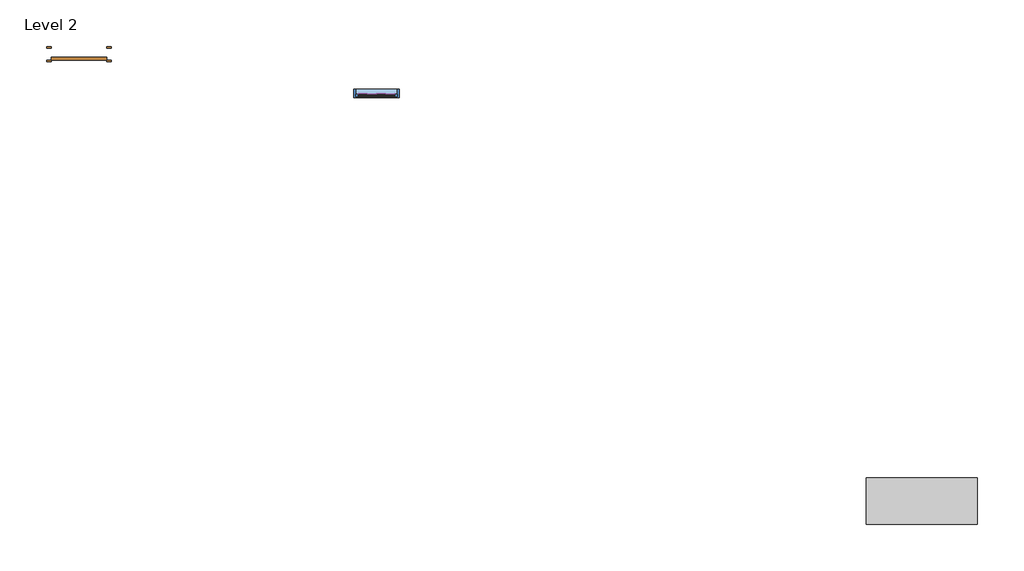
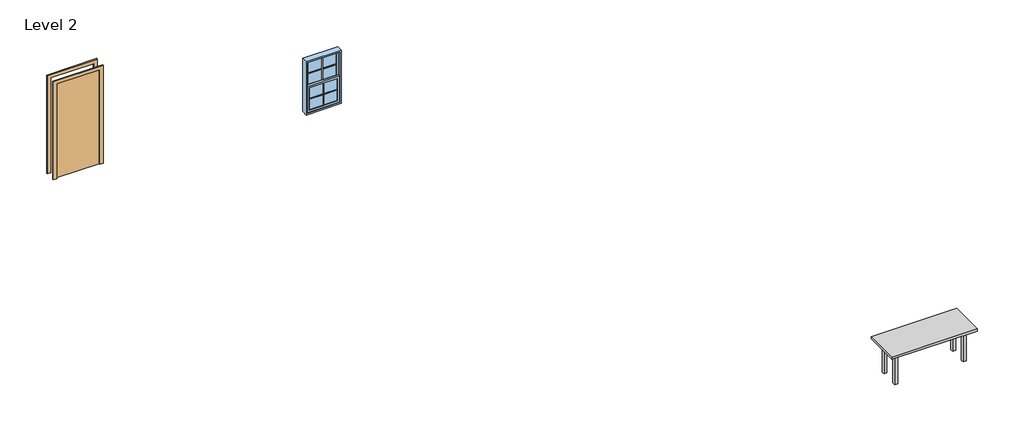
# One storey: 2 proxies, 1 door, 1 furniture element, 1 window.
"""IFC4 building model written with IfcOpenShell, lengths in millimetres."""

import ifcopenshell
import ifcopenshell.guid

model = None  # the IFC model being written
_history = None  # IfcOwnerHistory: only IFC2X3 demands one
_inside = {}  # id of a spatial element -> (the spatial element, [elements in it])
_under = {}  # id of a project, library or spatial element -> (it, [spatial elements below it])
_declared = {}  # id of a project -> (the project, [libraries it declares])
_typed = {}  # id of a type object -> (the type object, [elements of that type])
_made_of = {}  # id of a material, layer set ... -> (it, [elements and type objects made of it])


def new_model(schema):
    """Start an empty IFC model of exactly this schema.

    Asked for "IFC4X3", IfcOpenShell would pick the latest addendum, in which some entities
    have other attributes; the version numbers below select the first issue.
    IFC2X3 requires an IfcOwnerHistory on every rooted entity: one is made here for all.
    """
    global model, _history
    if schema == "IFC4X3":
        model = ifcopenshell.file(schema_version=(4, 3, 0, 0))
    else:
        model = ifcopenshell.file(schema=schema)
    _inside.clear()
    _under.clear()
    _declared.clear()
    _typed.clear()
    _made_of.clear()
    _history = None
    if model.schema == "IFC2X3":
        org = make("IfcOrganization", Name="unknown")
        user = make(
            "IfcPersonAndOrganization",
            ThePerson=make("IfcPerson", FamilyName="unknown"),
            TheOrganization=org,
        )
        app = make(
            "IfcApplication",
            ApplicationDeveloper=org,
            Version="unknown",
            ApplicationFullName="unknown",
            ApplicationIdentifier="unknown",
        )
        _history = make(
            "IfcOwnerHistory",
            OwningUser=user,
            OwningApplication=app,
            ChangeAction="ADDED",
            CreationDate=0,
        )
    return model


def make(cls, **values):
    """One entity of the class cls with the attributes given. An attribute that is None is left unset."""
    return model.create_entity(
        cls, **{name: value for name, value in values.items() if value is not None}
    )


def rooted(cls, **values):
    """An entity with a GlobalId (a new one), such as an element, a storey or a relation."""
    return make(cls, GlobalId=ifcopenshell.guid.new(), OwnerHistory=_history, **values)


def si_unit(unit_type, name, prefix=None):
    """IfcSIUnit, for example si_unit("LENGTHUNIT", "METRE", prefix="MILLI")."""
    return make("IfcSIUnit", UnitType=unit_type, Prefix=prefix, Name=name)


def assignment(units):
    """IfcUnitAssignment: the units of a project."""
    return None if units is None else make("IfcUnitAssignment", Units=units)


def point(xyz):
    """IfcCartesianPoint."""
    return None if xyz is None else make("IfcCartesianPoint", Coordinates=xyz)


def direction(xyz):
    """IfcDirection."""
    return None if xyz is None else make("IfcDirection", DirectionRatios=xyz)


def frame(location, z_axis=None, x_axis=None):
    """IfcAxis2Placement3D, a coordinate frame: its origin and axes. An axis left out is left unset."""
    return make(
        "IfcAxis2Placement3D",
        Location=point(location),
        Axis=direction(z_axis),
        RefDirection=direction(x_axis),
    )


def origin():
    """The frame at (0, 0, 0) with its axes left unset."""
    return frame((0.0, 0.0, 0.0))


def origin_with_axes():
    """The frame at (0, 0, 0) with the z axis (0, 0, 1) and the x axis (1, 0, 0) written out."""
    return frame((0.0, 0.0, 0.0), z_axis=(0.0, 0.0, 1.0), x_axis=(1.0, 0.0, 0.0))


def place(relative_to, where):
    """IfcLocalPlacement: puts the frame where relative to a parent placement (None: the world)."""
    return make(
        "IfcLocalPlacement", PlacementRelTo=relative_to, RelativePlacement=where
    )


def context(
    kind, dimensions, precision=None, world=None, true_north=None, identifier=None
):
    """IfcGeometricRepresentationContext, for example the 3D "Model" context."""
    return make(
        "IfcGeometricRepresentationContext",
        ContextIdentifier=identifier,
        ContextType=kind,
        CoordinateSpaceDimension=dimensions,
        Precision=precision,
        WorldCoordinateSystem=world,
        TrueNorth=true_north,
    )


def project(units=None, contexts=None):
    """IfcProject with its units and contexts."""
    return rooted(
        "IfcProject",
        Name="project",
        RepresentationContexts=contexts,
        UnitsInContext=assignment(units),
    )


def spatial(cls, under=None, at=None, **own):
    """A site, building, storey or space (cls), placed at a placement, below another one or the project."""
    s = rooted(cls, ObjectPlacement=at, **own)
    if under is not None:
        _under.setdefault(under.id(), (under, []))[1].append(s)
    return s


def polyline(points):
    """IfcPolyline through the points."""
    return make("IfcPolyline", Points=[point(p) for p in points])


def outline(outer, holes=None, kind="AREA"):
    """IfcArbitraryClosedProfileDef: a profile drawn as a closed curve; with holes, ...WithVoids."""
    if holes is None:
        return make("IfcArbitraryClosedProfileDef", ProfileType=kind, OuterCurve=outer)
    return make(
        "IfcArbitraryProfileDefWithVoids",
        ProfileType=kind,
        OuterCurve=outer,
        InnerCurves=holes,
    )


def extrude(swept, where, along, depth):
    """IfcExtrudedAreaSolid: the profile swept, set in the frame where, extruded along a direction by depth."""
    return make(
        "IfcExtrudedAreaSolid",
        SweptArea=swept,
        Position=where,
        ExtrudedDirection=direction(along),
        Depth=depth,
    )


def shape(context_of_items, identifier, shape_type, items):
    """IfcShapeRepresentation: the items that make up one representation, for example the "Body"."""
    return make(
        "IfcShapeRepresentation",
        ContextOfItems=context_of_items,
        RepresentationIdentifier=identifier,
        RepresentationType=shape_type,
        Items=items,
    )


def source(mapping_origin, context_of_items, identifier, shape_type, items):
    """IfcRepresentationMap: a shape defined once, which mapped items show again and again."""
    return make(
        "IfcRepresentationMap",
        MappingOrigin=mapping_origin,
        MappedRepresentation=shape(context_of_items, identifier, shape_type, items),
    )


def transform(
    local_origin,
    x_axis=None,
    y_axis=None,
    z_axis=None,
    scale=None,
    scale2=None,
    scale3=None,
    uniform=True,
):
    """IfcCartesianTransformationOperator3D, or its non-uniform kind. x_axis, y_axis, z_axis: its Axis1, 2, 3."""
    if uniform:
        return make(
            "IfcCartesianTransformationOperator3D",
            Axis1=direction(x_axis),
            Axis2=direction(y_axis),
            LocalOrigin=point(local_origin),
            Scale=scale,
            Axis3=direction(z_axis),
        )
    return make(
        "IfcCartesianTransformationOperator3DnonUniform",
        Axis1=direction(x_axis),
        Axis2=direction(y_axis),
        LocalOrigin=point(local_origin),
        Scale=scale,
        Axis3=direction(z_axis),
        Scale2=scale2,
        Scale3=scale3,
    )


def mapped(mapping_source, mapping_target):
    """IfcMappedItem: shows the shape of a source again, moved by a transform."""
    return make(
        "IfcMappedItem", MappingSource=mapping_source, MappingTarget=mapping_target
    )


def made_of(thing, what):
    """Note that an element or type object is made of a material, layer set ...; save() writes the relation."""
    if what is not None:
        _made_of.setdefault(what.id(), (what, []))[1].append(thing)
    return thing


def element(
    cls,
    number,
    at=None,
    inside=None,
    cuts=None,
    type_object=None,
    material=None,
    context=None,
    identifier="Body",
    shape_type=None,
    held_by="IfcProductDefinitionShape",
    body=None,
    shapes=None,
    **own,
):
    """One element of the class cls, such as IfcWall. Its Tag is "e" and its number.

    at: its placement. inside: the storey or other place that contains it. cuts: it is an
    opening in that element (IfcRelVoidsElement). A single representation is given by context,
    identifier, shape_type and body (its items); several are given by shapes. held_by: the class
    of the entity that holds the representations. save() writes the other relations.
    """
    e = rooted(cls, Tag="e%d" % number, ObjectPlacement=at, **own)
    if body is not None:
        shapes = [shape(context, identifier, shape_type, body)]
    if shapes is not None:
        e.Representation = make(held_by, Representations=shapes)
    if inside is not None:
        _inside.setdefault(inside.id(), (inside, []))[1].append(e)
    if cuts is not None:
        rooted(
            "IfcRelVoidsElement", RelatingBuildingElement=cuts, RelatedOpeningElement=e
        )
    if type_object is not None:
        _typed.setdefault(type_object.id(), (type_object, []))[1].append(e)
    return made_of(e, material)


def aggregate(whole, parts):
    """IfcRelAggregates: a whole, such as a stair, and the parts it consists of."""
    return rooted("IfcRelAggregates", RelatingObject=whole, RelatedObjects=parts)


def save(model, path):
    """Write the relations noted so far, then the file.

    IfcRelAggregates (storeys below a building ...), IfcRelContainedInSpatialStructure (elements
    in a storey), IfcRelDefinesByType, IfcRelAssociatesMaterial and IfcRelDeclares: one each for
    every whole, place, type object, material and project.
    """
    for whole, parts in _under.values():
        aggregate(whole, parts)
    for where, things in _inside.values():
        rooted(
            "IfcRelContainedInSpatialStructure",
            RelatedElements=things,
            RelatingStructure=where,
        )
    for kind, things in _typed.values():
        rooted("IfcRelDefinesByType", RelatedObjects=things, RelatingType=kind)
    for what, things in _made_of.values():
        rooted("IfcRelAssociatesMaterial", RelatedObjects=things, RelatingMaterial=what)
    for by, libraries in _declared.values():
        rooted("IfcRelDeclares", RelatingContext=by, RelatedDefinitions=libraries)
    model.write(path)


def m_muntin_pattern_2x2_m_muntin_pattern_2x2_aaec3afb(model_context):
    return source(origin(), model_context, "Body", "SweptSolid", [
        extrude(outline(polyline([(257.1375, -6.35), (257.1375, -298.8), (244.4375, -298.8), (244.4375, -6.35), (0.0, -6.35), (0.0, 6.35), (244.4375, 6.35), (244.4375, 298.8), (257.1375, 298.8), (257.1375, 6.35), (501.575, 6.35), (501.575, -6.35), (257.1375, -6.35)])), frame((0.0, 9.525, 0.0), z_axis=(0.0, 1.0, 0.0), x_axis=(0.0, 0.0, 1.0)), (0.0, 0.0, 1.0), 12.7),
        extrude(outline(polyline([(257.1375, -6.35), (257.1375, -298.8), (244.4375, -298.8), (244.4375, -6.35), (0.0, -6.35), (0.0, 6.35), (244.4375, 6.35), (244.4375, 298.8), (257.1375, 298.8), (257.1375, 6.35), (501.575, 6.35), (501.575, -6.35), (257.1375, -6.35)])), frame((0.0, -22.225, 0.0), z_axis=(0.0, 1.0, 0.0), x_axis=(0.0, 0.0, 1.0)), (0.0, 0.0, 1.0), 12.7),
    ])


def m_single_flush_0915_x_2134mm_6a9e8738(model_context):
    return source(origin(), model_context, "Body", "SweptSolid", [
        extrude(outline(polyline([(2210.0, -533.5), (0.0, -533.5), (0.0, -457.5), (2134.0, -457.5), (2134.0, 457.5), (0.0, 457.5), (0.0, 533.5), (2210.0, 533.5), (2210.0, -533.5)])), frame((0.0, 100.0, 0.0), z_axis=(0.0, 1.0, 0.0), x_axis=(0.0, 0.0, 1.0)), (0.0, 0.0, 1.0), 25.0),
        extrude(outline(polyline([(2210.0, 533.5), (2210.0, -533.5), (0.0, -533.5), (0.0, -457.5), (2134.0, -457.5), (2134.0, 457.5), (0.0, 457.5), (0.0, 533.5), (2210.0, 533.5)])), frame((0.0, -125.0, 0.0), z_axis=(0.0, 1.0, 0.0), x_axis=(0.0, 0.0, 1.0)), (0.0, 0.0, 1.0), 25.0),
        extrude(outline(polyline([(457.5, 49.0), (-457.5, 49.0), (-457.5, 100.0), (457.5, 100.0), (457.5, 49.0)])), origin_with_axes(), (0.0, 0.0, 1.0), 2134.0),
    ])


def m_table_rectangular_1830_x_0762mm_a0b3b7a0(model_context):
    return source(origin(), model_context, "Body", "SweptSolid", [
        extrude(outline(polyline([(699.1, 190.5), (699.1, 165.1), (-699.1, 165.1), (-699.1, 190.5), (699.1, 190.5)])), frame((0.0, 0.0, 609.6), z_axis=(0.0, 0.0, 1.0), x_axis=(1.0, 0.0, 0.0)), (0.0, 0.0, 1.0), 101.6),
        extrude(outline(polyline([(699.1, -190.5), (-699.1, -190.5), (-699.1, -165.1), (699.1, -165.1), (699.1, -190.5)])), frame((0.0, 0.0, 609.6), z_axis=(0.0, 0.0, 1.0), x_axis=(1.0, 0.0, 0.0)), (0.0, 0.0, 1.0), 101.6),
        extrude(outline(polyline([(-711.8, -165.1), (-737.2, -165.1), (-737.2, 165.1), (-711.8, 165.1), (-711.8, -165.1)])), frame((0.0, 0.0, 609.6), z_axis=(0.0, 0.0, 1.0), x_axis=(1.0, 0.0, 0.0)), (0.0, 0.0, 1.0), 101.6),
        extrude(outline(polyline([(711.8, -165.1), (711.8, 165.1), (737.2, 165.1), (737.2, -165.1), (711.8, -165.1)])), frame((0.0, 0.0, 609.6), z_axis=(0.0, 0.0, 1.0), x_axis=(1.0, 0.0, 0.0)), (0.0, 0.0, 1.0), 101.6),
        extrude(outline(polyline([(915.0, 381.0), (915.0, -381.0), (-915.0, -381.0), (-915.0, 381.0), (915.0, 381.0)])), frame((0.0, 0.0, 711.2), z_axis=(0.0, 0.0, 1.0), x_axis=(1.0, 0.0, 0.0)), (0.0, 0.0, 1.0), 50.8),
        extrude(outline(polyline([(-699.1, 228.6), (-699.1, 165.1), (-762.6, 165.1), (-762.6, 228.6), (-699.1, 228.6)])), origin_with_axes(), (0.0, 0.0, 1.0), 711.2),
        extrude(outline(polyline([(699.1, 228.6), (762.6, 228.6), (762.6, 165.1), (699.1, 165.1), (699.1, 228.6)])), origin_with_axes(), (0.0, 0.0, 1.0), 711.2),
        extrude(outline(polyline([(-699.1, -228.6), (-762.6, -228.6), (-762.6, -165.1), (-699.1, -165.1), (-699.1, -228.6)])), origin_with_axes(), (0.0, 0.0, 1.0), 711.2),
        extrude(outline(polyline([(699.1, -228.6), (699.1, -165.1), (762.6, -165.1), (762.6, -228.6), (699.1, -228.6)])), origin_with_axes(), (0.0, 0.0, 1.0), 711.2),
    ])


def m_window_double_hung_750_x_1200mm_e7ea5f28(model_context):
    return source(origin(), model_context, "Body", "SweptSolid", [
        extrude(outline(polyline([(298.8, -669.85), (298.8, -676.2), (-298.8, -676.2), (-298.8, -669.85), (298.8, -669.85)])), frame((0.0, 0.0, 990.6), z_axis=(0.0, 0.0, 1.0), x_axis=(1.0, 0.0, 0.0)), (0.0, 0.0, 1.0), 501.575),
        extrude(outline(polyline([(-298.8, -682.55), (298.8, -682.55), (298.8, -688.9), (-298.8, -688.9), (-298.8, -682.55)])), frame((0.0, 0.0, 990.6), z_axis=(0.0, 0.0, 1.0), x_axis=(1.0, 0.0, 0.0)), (0.0, 0.0, 1.0), 501.575),
        extrude(outline(polyline([(298.8, -625.4), (298.8, -631.75), (-298.8, -631.75), (-298.8, -625.4), (298.8, -625.4)])), frame((0.0, 0.0, 1536.625), z_axis=(0.0, 0.0, 1.0), x_axis=(1.0, 0.0, 0.0)), (0.0, 0.0, 1.0), 501.575),
        extrude(outline(polyline([(-298.8, -638.1), (298.8, -638.1), (298.8, -644.45), (-298.8, -644.45), (-298.8, -638.1)])), frame((0.0, 0.0, 1536.625), z_axis=(0.0, 0.0, 1.0), x_axis=(1.0, 0.0, 0.0)), (0.0, 0.0, 1.0), 501.575),
        extrude(outline(polyline([(1536.625, -343.25), (946.15, -343.25), (946.15, 343.25), (1536.625, 343.25), (1536.625, -343.25)]), holes=[polyline([(1492.175, 298.8), (990.6, 298.8), (990.6, -298.8), (1492.175, -298.8), (1492.175, 298.8)])]), frame((0.0, -701.6, 0.0), z_axis=(0.0, 1.0, 0.0), x_axis=(0.0, 0.0, 1.0)), (0.0, 0.0, 1.0), 44.45),
        extrude(outline(polyline([(2082.65, -343.25), (1492.175, -343.25), (1492.175, 343.25), (2082.65, 343.25), (2082.65, -343.25)]), holes=[polyline([(2038.2, 298.8), (1536.625, 298.8), (1536.625, -298.8), (2038.2, -298.8), (2038.2, 298.8)])]), frame((0.0, -657.15, 0.0), z_axis=(0.0, 1.0, 0.0), x_axis=(0.0, 0.0, 1.0)), (0.0, 0.0, 1.0), 44.45),
        extrude(outline(polyline([(2114.4, -375.0), (914.4, -375.0), (914.4, 375.0), (2114.4, 375.0), (2114.4, -375.0)]), holes=[polyline([(2082.65, 343.25), (946.15, 343.25), (946.15, -343.25), (2082.65, -343.25), (2082.65, 343.25)])]), frame((0.0, -714.3, 0.0), z_axis=(0.0, 1.0, 0.0), x_axis=(0.0, 0.0, 1.0)), (0.0, 0.0, 1.0), 133.35),
    ])


model = new_model("IFC4")

# Units and contexts
model_context = context("Model", 3, world=origin())
ifc_project = project(units=[si_unit("LENGTHUNIT", "METRE", prefix="MILLI")], contexts=[model_context])

# Site, building, storey
site = spatial("IfcSite", under=ifc_project)
building = spatial("IfcBuilding", under=site)
storey = spatial("IfcBuildingStorey", under=building, Name="Level 2", Elevation=4000.0)

# Proxies
placement = place(None, origin())
m_muntin_pattern_2x2_m_muntin_pattern_2x2_shape = m_muntin_pattern_2x2_m_muntin_pattern_2x2_aaec3afb(model_context)
element("IfcBuildingElementProxy", 1, Name="M_Muntin Pattern_2x2 : M_Muntin Pattern_2x2", ObjectType="M_Muntin Pattern_2x2 : M_Muntin Pattern_2x2", at=placement, inside=storey, context=model_context, shape_type="MappedRepresentation", body=[
    mapped(m_muntin_pattern_2x2_m_muntin_pattern_2x2_shape, transform((-15264.9853759, 1399.5505832, 5536.625), x_axis=(1.0, 0.0, 0.0), y_axis=(0.0, 1.0, 0.0), z_axis=(0.0, 0.0, 1.0))),
])
element("IfcBuildingElementProxy", 2, Name="M_Muntin Pattern_2x2 : M_Muntin Pattern_2x2", ObjectType="M_Muntin Pattern_2x2 : M_Muntin Pattern_2x2", at=placement, inside=storey, context=model_context, shape_type="MappedRepresentation", body=[
    mapped(m_muntin_pattern_2x2_m_muntin_pattern_2x2_shape, transform((-15264.9853759, 1355.1005832, 4990.6), x_axis=(1.0, 0.0, 0.0), y_axis=(0.0, 1.0, 0.0), z_axis=(0.0, 0.0, 1.0))),
])

# Door
m_single_flush_0915_x_2134mm_shape = m_single_flush_0915_x_2134mm_6a9e8738(model_context)
element("IfcDoor", 3, ObjectType="M_Single-Flush : 0915 x 2134mm", at=placement, inside=storey, context=model_context, shape_type="MappedRepresentation", body=[
    mapped(m_single_flush_0915_x_2134mm_shape, transform((-20159.8897659, 2034.4755832, 4866.0), x_axis=(-1.0, 0.0, 0.0), y_axis=(0.0, -1.0, 0.0), z_axis=(0.0, 0.0, 1.0))),
])

# Furniture
m_table_rectangular_1830_x_0762mm_shape = m_table_rectangular_1830_x_0762mm_a0b3b7a0(model_context)
element("IfcFurniture", 4, ObjectType="M_Table-Rectangular : 1830 x 0762mm", at=placement, inside=storey, context=model_context, shape_type="MappedRepresentation", body=[
    mapped(m_table_rectangular_1830_x_0762mm_shape, transform((-6296.1972949, -5323.9774044, 0.0), x_axis=(-1.0, 0.0, 0.0), y_axis=(0.0, -1.0, 0.0), z_axis=(0.0, 0.0, 1.0))),
])

# Window
m_window_double_hung_750_x_1200mm_shape = m_window_double_hung_750_x_1200mm_e7ea5f28(model_context)
element("IfcWindow", 5, ObjectType="M_Window-Double-Hung : 750 x 1200mm", at=placement, inside=storey, context=model_context, shape_type="MappedRepresentation", body=[
    mapped(m_window_double_hung_750_x_1200mm_shape, transform((-15264.9853759, 2034.4755832, 4000.0), x_axis=(1.0, 0.0, 0.0), y_axis=(0.0, 1.0, 0.0), z_axis=(0.0, 0.0, 1.0))),
])

save(model, "model.ifc")

# Revit data of these elements
# Type "M_Muntin Pattern_2x2 : M_Muntin Pattern_2x2"
#   Width [instance default] = 1200 mm
#   Thickness = 12.7 mm
#   Height [instance default] = 1200 mm
#   Distance = 19.05 mm
#   Interior Material [instance default] = none
#   Exterior Material [instance default] = none
#   Default Elevation = 0
# Type "M_Single-Flush : 0915 x 2134mm"
#   Type Mark = "20"
#   Construction Type Id = "MDOOR"
#   Analytic Construction = "Metal"
#   Thickness = 51 mm
#   Thermal Resistance (R) = 0.270117 (m²·K)/W
#   Heat Transfer Coefficient (U) = 3.7021 W/(m²·K)
#   Height = 2134 mm
#   Trim Projection Ext = 25 mm
#   Trim Projection Int = 25 mm
#   Trim Width = 76 mm
#   Width = 915 mm
#   Define Thermal Properties by = 1
#   Define Thermal Properties by = 1
#   Door Material = Door - Panel
#   Frame Material = Door - Frame
#   Visual Light Transmittance = 0
#   Solar Heat Gain Coefficient = 0
#   Function = (empty or 0)
#   Wall Closure = (empty or 0)
# Type "M_Table-Rectangular : 1830 x 0762mm"
#   Height = 762 mm
#   Length = 1830 mm
#   Width = 762 mm
#   Base Material = Birch
#   Top Material = Birch
#   Default Elevation = 0
# Type "M_Window-Double-Hung : 750 x 1200mm"
#   Type Mark = "22"
#   Fire Rating = "0.5h"
#   Construction Type Id = "DG-DR"
#   Assembly Code = "B2020100"
#   Analytic Construction = "Double glazing - domestic"
#   Wall Thickness [instance default] = 150 mm
#   Window Inset [instance default] = 0 mm
#   Visual Light Transmittance = 0.81
#   Thermal Resistance (R) = 0.319569 (m²·K)/W
#   Solar Heat Gain Coefficient = 0.76
#   Muntin Width = 597.6 mm
#   Muntin Height = 501.575 mm
#   Interior Wall Closure [instance default] = 35.7 mm
#   Rough Width = 765 mm
#   Rough Height = 1215 mm
#   Frame Extension [instance default] = 31.75 mm
#   Exterior Wall Closure [instance default] = 12.7 mm
#   Extension Jamb [instance default] = 35.7 mm
#   Heat Transfer Coefficient (U) = 3.12929 W/(m²·K)
#   Height = 1200 mm
#   Width = 750 mm
#   Define Thermal Properties by = 1
#   Top Muntin Visibility = yes
#   Indicator Visibility [instance default] = yes
#   Extension Jamb Visibility [instance default] = yes
#   Interior Trim Visibility [instance default] = yes
#   Exterior Trim Visibility [instance default] = yes
#   Define Thermal Properties by = 1
#   Bottom Muntin Visibility = yes
#   Muntin Pattern = M_Muntin Pattern_2x2 : M_Muntin Pattern_2x2
#   Interior Trim Material = Wood - Stained
#   Interior Trim = M_Trim-Window-Interior-Flat : Picture Frame
#   Exterior Trim Material = Clad - White
#   Exterior Trim = M_Trim-Window-Exterior-Flat : with Sill
#   Glass Panel Material = Glass
#   Exterior Frame Material = Clad - White
#   Interior Frame Material = Wood - Stained
#   Wall Closure = (empty or 0)
# Elements 1, 2 (IfcBuildingElementProxy, "M_Muntin Pattern_2x2 : M_Muntin Pattern_2x2")
#   Width = 597.6 mm
#   Height = 501.575 mm
#   Interior Material = Wood - Stained
#   Exterior Material = Clad - White
#   Phase Created = New Construction
#   Materials on its faces: "Clad - White", "Wood - Stained"
# Element 3 (IfcDoor, "M_Single-Flush : 0915 x 2134mm")
#   SpeckleObjectTestNumber = 5
#   Phase Created = New Construction
#   Materials on its faces: "Door - Frame", "Door - Panel"
# Element 4 (IfcFurniture, "M_Table-Rectangular : 1830 x 0762mm")
#   SpeckleObjectTestNumber = 10
#   Phase Created = New Construction
#   Materials on its faces: "Birch"
# Element 5 (IfcWindow, "M_Window-Double-Hung : 750 x 1200mm")
#   Mark = "4"
#   Window Inset = 700 mm
#   Interior Wall Closure = 60 mm
#   Frame Extension = 31.75 mm
#   Exterior Wall Closure = 50 mm
#   SpeckleObjectTestNumber = 7
#   Interior Trim Visibility = no
#   Indicator Visibility = no
#   Exterior Trim Visibility = no
#   Phase Created = New Construction
#   Materials on its faces: "Wood - Stained", "Glass", "Clad - White"
# Materials
#   "Door - Panel": class "Wood", colour RGB 210 159 95, transparency 0, Cost = 0
#   "Door - Frame": class "Miscellaneous", colour RGB 118 70 51, transparency 0, Cost = 0
#   "Birch": class "Wood", colour RGB 224 178 126, transparency 0, Description = "Betula Alleghaniensis", Cost = 0
#   "Wood - Stained": class "Wood", colour RGB 224 178 126, transparency 0, Cost = 0
#   "Clad - White": class "Wood", colour RGB 242 242 238, transparency 0, Cost = 0
#   "Glass": class "Glass", colour RGB 0 128 192, transparency 0.9, Description = "Soda Lime Glass", Cost = 0
